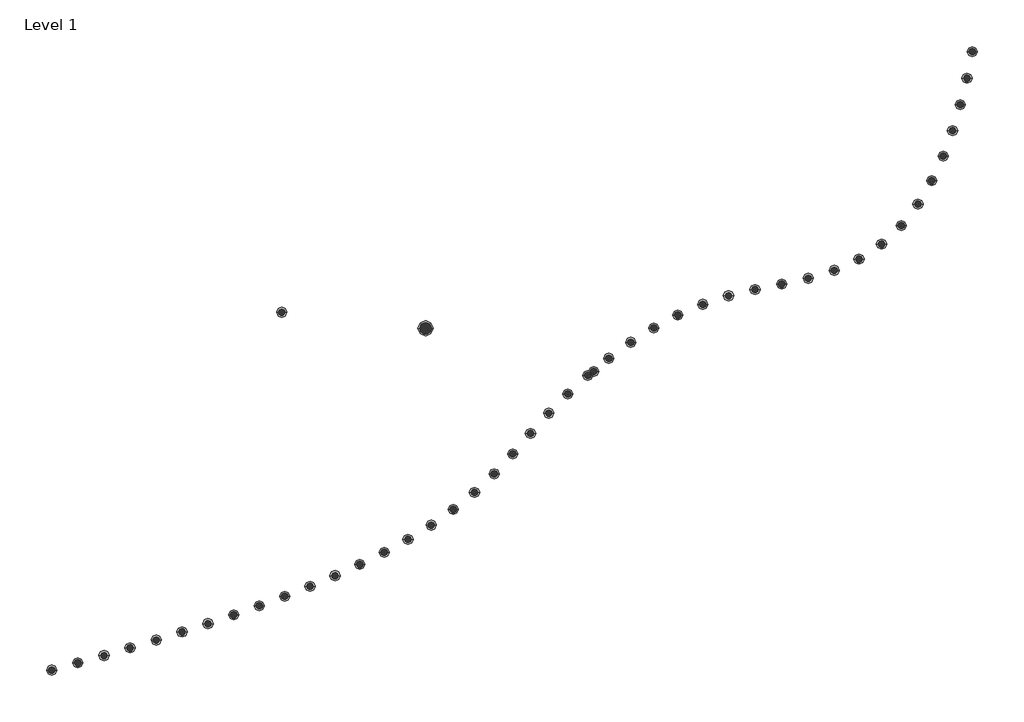
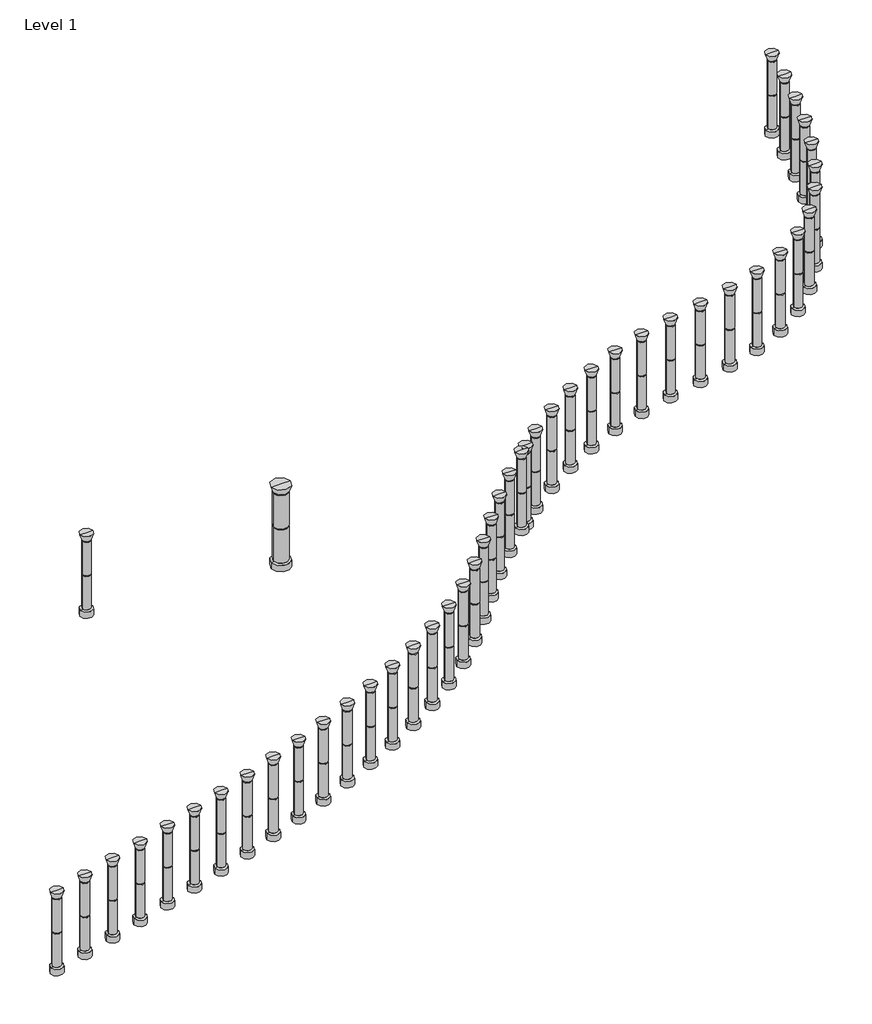
# One storey: 47 columns.
"""IFC4 building model written with IfcOpenShell, lengths in millimetres."""

import ifcopenshell
import ifcopenshell.guid

model = None  # the IFC model being written
_history = None  # IfcOwnerHistory: only IFC2X3 demands one
_inside = {}  # id of a spatial element -> (the spatial element, [elements in it])
_under = {}  # id of a project, library or spatial element -> (it, [spatial elements below it])
_declared = {}  # id of a project -> (the project, [libraries it declares])
_typed = {}  # id of a type object -> (the type object, [elements of that type])
_made_of = {}  # id of a material, layer set ... -> (it, [elements and type objects made of it])


def new_model(schema):
    """Start an empty IFC model of exactly this schema.

    Asked for "IFC4X3", IfcOpenShell would pick the latest addendum, in which some entities
    have other attributes; the version numbers below select the first issue.
    IFC2X3 requires an IfcOwnerHistory on every rooted entity: one is made here for all.
    """
    global model, _history
    if schema == "IFC4X3":
        model = ifcopenshell.file(schema_version=(4, 3, 0, 0))
    else:
        model = ifcopenshell.file(schema=schema)
    _inside.clear()
    _under.clear()
    _declared.clear()
    _typed.clear()
    _made_of.clear()
    _history = None
    if model.schema == "IFC2X3":
        org = make("IfcOrganization", Name="unknown")
        user = make(
            "IfcPersonAndOrganization",
            ThePerson=make("IfcPerson", FamilyName="unknown"),
            TheOrganization=org,
        )
        app = make(
            "IfcApplication",
            ApplicationDeveloper=org,
            Version="unknown",
            ApplicationFullName="unknown",
            ApplicationIdentifier="unknown",
        )
        _history = make(
            "IfcOwnerHistory",
            OwningUser=user,
            OwningApplication=app,
            ChangeAction="ADDED",
            CreationDate=0,
        )
    return model


def make(cls, **values):
    """One entity of the class cls with the attributes given. An attribute that is None is left unset."""
    return model.create_entity(
        cls, **{name: value for name, value in values.items() if value is not None}
    )


def rooted(cls, **values):
    """An entity with a GlobalId (a new one), such as an element, a storey or a relation."""
    return make(cls, GlobalId=ifcopenshell.guid.new(), OwnerHistory=_history, **values)


def si_unit(unit_type, name, prefix=None):
    """IfcSIUnit, for example si_unit("LENGTHUNIT", "METRE", prefix="MILLI")."""
    return make("IfcSIUnit", UnitType=unit_type, Prefix=prefix, Name=name)


def assignment(units):
    """IfcUnitAssignment: the units of a project."""
    return None if units is None else make("IfcUnitAssignment", Units=units)


def point(xyz):
    """IfcCartesianPoint."""
    return None if xyz is None else make("IfcCartesianPoint", Coordinates=xyz)


def direction(xyz):
    """IfcDirection."""
    return None if xyz is None else make("IfcDirection", DirectionRatios=xyz)


def frame(location, z_axis=None, x_axis=None):
    """IfcAxis2Placement3D, a coordinate frame: its origin and axes. An axis left out is left unset."""
    return make(
        "IfcAxis2Placement3D",
        Location=point(location),
        Axis=direction(z_axis),
        RefDirection=direction(x_axis),
    )


def origin():
    """The frame at (0, 0, 0) with its axes left unset."""
    return frame((0.0, 0.0, 0.0))


def origin_with_axes():
    """The frame at (0, 0, 0) with the z axis (0, 0, 1) and the x axis (1, 0, 0) written out."""
    return frame((0.0, 0.0, 0.0), z_axis=(0.0, 0.0, 1.0), x_axis=(1.0, 0.0, 0.0))


def place(relative_to, where):
    """IfcLocalPlacement: puts the frame where relative to a parent placement (None: the world)."""
    return make(
        "IfcLocalPlacement", PlacementRelTo=relative_to, RelativePlacement=where
    )


def context(
    kind, dimensions, precision=None, world=None, true_north=None, identifier=None
):
    """IfcGeometricRepresentationContext, for example the 3D "Model" context."""
    return make(
        "IfcGeometricRepresentationContext",
        ContextIdentifier=identifier,
        ContextType=kind,
        CoordinateSpaceDimension=dimensions,
        Precision=precision,
        WorldCoordinateSystem=world,
        TrueNorth=true_north,
    )


def project(units=None, contexts=None):
    """IfcProject with its units and contexts."""
    return rooted(
        "IfcProject",
        Name="project",
        RepresentationContexts=contexts,
        UnitsInContext=assignment(units),
    )


def spatial(cls, under=None, at=None, **own):
    """A site, building, storey or space (cls), placed at a placement, below another one or the project."""
    s = rooted(cls, ObjectPlacement=at, **own)
    if under is not None:
        _under.setdefault(under.id(), (under, []))[1].append(s)
    return s


def polyline(points):
    """IfcPolyline through the points."""
    return make("IfcPolyline", Points=[point(p) for p in points])


def circle_curve(where, radius):
    """IfcCircle in the frame where."""
    return make("IfcCircle", Position=where, Radius=radius)


def shape(context_of_items, identifier, shape_type, items):
    """IfcShapeRepresentation: the items that make up one representation, for example the "Body"."""
    return make(
        "IfcShapeRepresentation",
        ContextOfItems=context_of_items,
        RepresentationIdentifier=identifier,
        RepresentationType=shape_type,
        Items=items,
    )


def source(mapping_origin, context_of_items, identifier, shape_type, items):
    """IfcRepresentationMap: a shape defined once, which mapped items show again and again."""
    return make(
        "IfcRepresentationMap",
        MappingOrigin=mapping_origin,
        MappedRepresentation=shape(context_of_items, identifier, shape_type, items),
    )


def transform(
    local_origin,
    x_axis=None,
    y_axis=None,
    z_axis=None,
    scale=None,
    scale2=None,
    scale3=None,
    uniform=True,
):
    """IfcCartesianTransformationOperator3D, or its non-uniform kind. x_axis, y_axis, z_axis: its Axis1, 2, 3."""
    if uniform:
        return make(
            "IfcCartesianTransformationOperator3D",
            Axis1=direction(x_axis),
            Axis2=direction(y_axis),
            LocalOrigin=point(local_origin),
            Scale=scale,
            Axis3=direction(z_axis),
        )
    return make(
        "IfcCartesianTransformationOperator3DnonUniform",
        Axis1=direction(x_axis),
        Axis2=direction(y_axis),
        LocalOrigin=point(local_origin),
        Scale=scale,
        Axis3=direction(z_axis),
        Scale2=scale2,
        Scale3=scale3,
    )


def mapped(mapping_source, mapping_target):
    """IfcMappedItem: shows the shape of a source again, moved by a transform."""
    return make(
        "IfcMappedItem", MappingSource=mapping_source, MappingTarget=mapping_target
    )


def made_of(thing, what):
    """Note that an element or type object is made of a material, layer set ...; save() writes the relation."""
    if what is not None:
        _made_of.setdefault(what.id(), (what, []))[1].append(thing)
    return thing


def element(
    cls,
    number,
    at=None,
    inside=None,
    cuts=None,
    type_object=None,
    material=None,
    context=None,
    identifier="Body",
    shape_type=None,
    held_by="IfcProductDefinitionShape",
    body=None,
    shapes=None,
    **own,
):
    """One element of the class cls, such as IfcWall. Its Tag is "e" and its number.

    at: its placement. inside: the storey or other place that contains it. cuts: it is an
    opening in that element (IfcRelVoidsElement). A single representation is given by context,
    identifier, shape_type and body (its items); several are given by shapes. held_by: the class
    of the entity that holds the representations. save() writes the other relations.
    """
    e = rooted(cls, Tag="e%d" % number, ObjectPlacement=at, **own)
    if body is not None:
        shapes = [shape(context, identifier, shape_type, body)]
    if shapes is not None:
        e.Representation = make(held_by, Representations=shapes)
    if inside is not None:
        _inside.setdefault(inside.id(), (inside, []))[1].append(e)
    if cuts is not None:
        rooted(
            "IfcRelVoidsElement", RelatingBuildingElement=cuts, RelatedOpeningElement=e
        )
    if type_object is not None:
        _typed.setdefault(type_object.id(), (type_object, []))[1].append(e)
    return made_of(e, material)


def aggregate(whole, parts):
    """IfcRelAggregates: a whole, such as a stair, and the parts it consists of."""
    return rooted("IfcRelAggregates", RelatingObject=whole, RelatedObjects=parts)


def save(model, path):
    """Write the relations noted so far, then the file.

    IfcRelAggregates (storeys below a building ...), IfcRelContainedInSpatialStructure (elements
    in a storey), IfcRelDefinesByType, IfcRelAssociatesMaterial and IfcRelDeclares: one each for
    every whole, place, type object, material and project.
    """
    for whole, parts in _under.values():
        aggregate(whole, parts)
    for where, things in _inside.values():
        rooted(
            "IfcRelContainedInSpatialStructure",
            RelatedElements=things,
            RelatingStructure=where,
        )
    for kind, things in _typed.values():
        rooted("IfcRelDefinesByType", RelatedObjects=things, RelatingType=kind)
    for what, things in _made_of.values():
        rooted("IfcRelAssociatesMaterial", RelatedObjects=things, RelatingMaterial=what)
    for by, libraries in _declared.values():
        rooted("IfcRelDeclares", RelatingContext=by, RelatedDefinitions=libraries)
    model.write(path)


def plane_surface(at):
    """IfcPlane: the flat surface through the origin of the frame at, square to its z axis."""
    return make("IfcPlane", Position=at)


def cylinder_surface(at, radius):
    """IfcCylindricalSurface: all points at the distance radius from the z axis of the frame at."""
    return make("IfcCylindricalSurface", Position=at, Radius=radius)


def revolved_surface(curve, axis_point, axis_direction):
    """IfcSurfaceOfRevolution: the curve turned about the line through axis_point along axis_direction."""
    return make(
        "IfcSurfaceOfRevolution",
        SweptCurve=make("IfcArbitraryOpenProfileDef", ProfileType="CURVE", Curve=curve),
        AxisPosition=make("IfcAxis1Placement", Location=point(axis_point), Axis=direction(axis_direction)),
    )


def advanced_brep(points, edges, surfaces, faces):
    """IfcAdvancedBrep: a solid bounded by faces that lie on surfaces and meet in shared edges.

    An edge is (start, end): straight between two places in points (the first is 0);
    or (start, end, curve); or (start, end, curve, False) where it runs against its curve.
    A face is (place in surfaces, loops), or (place, loops, False) where it looks against
    its surface's normal. A loop lists edges by number (the first is 1), with a minus sign
    where the edge is run from its end to its start. The first loop is the outer one.
    """
    corners = [point(p) for p in points]
    vertices = [make("IfcVertexPoint", VertexGeometry=c) for c in corners]
    made = []
    for start, end, *more in edges:
        made.append(
            make(
                "IfcEdgeCurve",
                EdgeStart=vertices[start],
                EdgeEnd=vertices[end],
                EdgeGeometry=more[0] if more else make("IfcPolyline", Points=[corners[start], corners[end]]),
                SameSense=more[1] if len(more) > 1 else True,
            )
        )
    hull = []
    for where, loops, *sense in faces:
        bounds = []
        for j, loop in enumerate(loops):
            ring = [make("IfcOrientedEdge", EdgeElement=made[abs(k) - 1], Orientation=k > 0) for k in loop]
            bounds.append(
                make(
                    "IfcFaceOuterBound" if j == 0 else "IfcFaceBound",
                    Bound=make("IfcEdgeLoop", EdgeList=ring),
                    Orientation=True,
                )
            )
        hull.append(make("IfcAdvancedFace", Bounds=bounds, FaceSurface=surfaces[where], SameSense=sense[0] if sense else True))
    return make("IfcAdvancedBrep", Outer=make("IfcClosedShell", CfsFaces=hull))


def column_with_capital_parametric_column_with_capital_56f4d1e8(model_context):
    return source(origin(), model_context, "Body", "AdvancedBrep", [
        advanced_brep(
        [(-300.0, 0.0, 300.0), (300.0, 0.0, 300.0), (300.0, 0.0, 0.0), (-300.0, 0.0, 0.0), (0.0, 0.0, 0.0), (-150.0, 0.0, 300.0), (150.0, 0.0, 300.0), (-150.0, 0.0, 350.0), (150.0, 0.0, 350.0), (-200.0, 0.0, 350.0), (200.0, 0.0, 350.0), (-200.0, 0.0, 1975.0), (200.0, 0.0, 1975.0), (0.0, 0.0, 4000.0), (300.0, 0.0, 4000.0), (-300.0, 0.0, 4000.0), (200.0, 0.0, 3700.0), (-200.0, 0.0, 3700.0), (-150.0, 0.0, 3650.0), (150.0, 0.0, 3650.0), (200.0, 0.0, 3650.0), (-200.0, 0.0, 3650.0), (200.0, 0.0, 2025.0), (-200.0, 0.0, 2025.0), (-150.0, 0.0, 3700.0), (150.0, 0.0, 3700.0), (-150.0, 0.0, 1975.0), (150.0, 0.0, 1975.0), (-150.0, 0.0, 2025.0), (150.0, 0.0, 2025.0)],
        [
            (0, 1, circle_curve(frame((0.0, 0.0, 300.0), z_axis=(0.0, 0.0, -1.0), x_axis=(1.0, 0.0, 0.0)), 300.0)),
            (1, 2),
            (2, 3, circle_curve(origin_with_axes(), 300.0)),
            (3, 0),
            (2, 4),
            (4, 3),
            (2, 3, circle_curve(frame((0.0, 0.0, 0.0), z_axis=(0.0, 0.0, -1.0), x_axis=(1.0, 0.0, 0.0)), 300.0)),
            (1, 0, circle_curve(frame((0.0, 0.0, 300.0), z_axis=(0.0, 0.0, -1.0), x_axis=(1.0, 0.0, 0.0)), 300.0)),
            (5, 6, circle_curve(frame((0.0, 0.0, 300.0), z_axis=(0.0, 0.0, -1.0), x_axis=(1.0, 0.0, 0.0)), 150.0)),
            (6, 1),
            (0, 5),
            (6, 5, circle_curve(frame((0.0, 0.0, 300.0), z_axis=(0.0, 0.0, -1.0), x_axis=(1.0, 0.0, 0.0)), 150.0)),
            (7, 8, circle_curve(frame((0.0, 0.0, 350.0), z_axis=(0.0, 0.0, -1.0), x_axis=(1.0, 0.0, 0.0)), 150.0)),
            (8, 6),
            (5, 7),
            (8, 7, circle_curve(frame((0.0, 0.0, 350.0), z_axis=(0.0, 0.0, -1.0), x_axis=(1.0, 0.0, 0.0)), 150.0)),
            (9, 10, circle_curve(frame((0.0, 0.0, 350.0), z_axis=(0.0, 0.0, -1.0), x_axis=(1.0, 0.0, 0.0)), 200.0)),
            (10, 8),
            (7, 9),
            (10, 9, circle_curve(frame((0.0, 0.0, 350.0), z_axis=(0.0, 0.0, -1.0), x_axis=(1.0, 0.0, 0.0)), 200.0)),
            (11, 12, circle_curve(frame((0.0, 0.0, 1975.0), z_axis=(0.0, 0.0, -1.0), x_axis=(1.0, 0.0, 0.0)), 200.0)),
            (12, 10),
            (9, 11),
            (12, 11, circle_curve(frame((0.0, 0.0, 1975.0), z_axis=(0.0, 0.0, -1.0), x_axis=(1.0, 0.0, 0.0)), 200.0)),
            (13, 14),
            (14, 15, circle_curve(frame((0.0, 0.0, 4000.0), z_axis=(0.0, 0.0, 1.0), x_axis=(1.0, 0.0, 0.0)), 300.0)),
            (15, 13),
            (15, 14, circle_curve(frame((0.0, 0.0, 4000.0), z_axis=(0.0, 0.0, 1.0), x_axis=(1.0, 0.0, 0.0)), 300.0)),
            (14, 16),
            (16, 17, circle_curve(frame((0.0, 0.0, 3700.0), z_axis=(0.0, 0.0, 1.0), x_axis=(1.0, 0.0, 0.0)), 200.0)),
            (17, 15),
            (17, 16, circle_curve(frame((0.0, 0.0, 3700.0), z_axis=(0.0, 0.0, 1.0), x_axis=(1.0, 0.0, 0.0)), 200.0)),
            (18, 19, circle_curve(frame((0.0, 0.0, 3650.0), z_axis=(0.0, 0.0, -1.0), x_axis=(1.0, 0.0, 0.0)), 150.0)),
            (19, 20),
            (20, 21, circle_curve(frame((0.0, 0.0, 3650.0), z_axis=(0.0, 0.0, 1.0), x_axis=(1.0, 0.0, 0.0)), 200.0)),
            (21, 18),
            (20, 22),
            (22, 23, circle_curve(frame((0.0, 0.0, 2025.0), z_axis=(0.0, 0.0, 1.0), x_axis=(1.0, 0.0, 0.0)), 200.0)),
            (23, 21),
            (20, 21, circle_curve(frame((0.0, 0.0, 3650.0), z_axis=(0.0, 0.0, -1.0), x_axis=(1.0, 0.0, 0.0)), 200.0)),
            (23, 22, circle_curve(frame((0.0, 0.0, 2025.0), z_axis=(0.0, 0.0, 1.0), x_axis=(1.0, 0.0, 0.0)), 200.0)),
            (19, 18, circle_curve(frame((0.0, 0.0, 3650.0), z_axis=(0.0, 0.0, -1.0), x_axis=(1.0, 0.0, 0.0)), 150.0)),
            (24, 25, circle_curve(frame((0.0, 0.0, 3700.0), z_axis=(0.0, 0.0, -1.0), x_axis=(1.0, 0.0, 0.0)), 150.0)),
            (25, 19),
            (18, 24),
            (25, 24, circle_curve(frame((0.0, 0.0, 3700.0), z_axis=(0.0, 0.0, -1.0), x_axis=(1.0, 0.0, 0.0)), 150.0)),
            (16, 25),
            (24, 17),
            (26, 27, circle_curve(frame((0.0, 0.0, 1975.0), z_axis=(0.0, 0.0, -1.0), x_axis=(1.0, 0.0, 0.0)), 150.0)),
            (27, 12),
            (11, 26),
            (27, 26, circle_curve(frame((0.0, 0.0, 1975.0), z_axis=(0.0, 0.0, -1.0), x_axis=(1.0, 0.0, 0.0)), 150.0)),
            (28, 29, circle_curve(frame((0.0, 0.0, 2025.0), z_axis=(0.0, 0.0, -1.0), x_axis=(1.0, 0.0, 0.0)), 150.0)),
            (29, 27),
            (26, 28),
            (29, 28, circle_curve(frame((0.0, 0.0, 2025.0), z_axis=(0.0, 0.0, -1.0), x_axis=(1.0, 0.0, 0.0)), 150.0)),
            (22, 29),
            (28, 23),
        ],
        [
            cylinder_surface(frame((0.0, 0.0, 4203.0565088), z_axis=(0.0, 0.0, 1.0), x_axis=(1.0, 0.0, 0.0)), 300.0),
            plane_surface(frame((0.0, 0.0, 0.0), z_axis=(0.0, 0.0, -1.0), x_axis=(1.0, 0.0, 0.0))),
            plane_surface(frame((0.0, 0.0, 300.0), z_axis=(0.0, 0.0, 1.0), x_axis=(1.0, 0.0, 0.0))),
            cylinder_surface(frame((0.0, 0.0, 4203.0565088), z_axis=(0.0, 0.0, 1.0), x_axis=(1.0, 0.0, 0.0)), 150.0),
            plane_surface(frame((0.0, 0.0, 350.0), z_axis=(0.0, 0.0, -1.0), x_axis=(1.0, 0.0, 0.0))),
            cylinder_surface(frame((0.0, 0.0, 4203.0565088), z_axis=(0.0, 0.0, 1.0), x_axis=(1.0, 0.0, 0.0)), 200.0),
            plane_surface(frame((0.0, 0.0, 4000.0), z_axis=(0.0, 0.0, 1.0), x_axis=(1.0, 0.0, 0.0))),
            revolved_surface(polyline([(200.0, 0.0, 3700.0), (300.0, 0.0, 4000.0)]), (0.0, 0.0, 4203.0565088), (0.0, 0.0, 1.0)),
            plane_surface(frame((0.0, 0.0, 3650.0), z_axis=(0.0, 0.0, 1.0), x_axis=(1.0, 0.0, 0.0))),
            plane_surface(frame((0.0, 0.0, 3700.0), z_axis=(0.0, 0.0, -1.0), x_axis=(1.0, 0.0, 0.0))),
            plane_surface(frame((0.0, 0.0, 1975.0), z_axis=(0.0, 0.0, 1.0), x_axis=(1.0, 0.0, 0.0))),
            plane_surface(frame((0.0, 0.0, 2025.0), z_axis=(0.0, 0.0, -1.0), x_axis=(1.0, 0.0, 0.0))),
        ],
        [
            (0, [[1, 2, 3, 4]]),
            (1, [[-3, 5, 6]]),
            (1, [[7, -6, -5]]),
            (0, [[8, -4, -7, -2]]),
            (2, [[9, 10, -1, 11]]),
            (2, [[12, -11, -8, -10]]),
            (3, [[13, 14, -9, 15]]),
            (3, [[16, -15, -12, -14]]),
            (4, [[17, 18, -13, 19]]),
            (4, [[20, -19, -16, -18]]),
            (5, [[21, 22, -17, 23]]),
            (5, [[24, -23, -20, -22]]),
            (6, [[25, 26, 27]]),
            (6, [[-27, 28, -25]]),
            (7, [[-26, 29, 30, 31]]),
            (7, [[-28, -31, 32, -29]]),
            (8, [[33, 34, 35, 36]]),
            (5, [[-35, 37, 38, 39]]),
            (5, [[40, -39, 41, -37]]),
            (8, [[42, -36, -40, -34]]),
            (3, [[43, 44, -33, 45]]),
            (3, [[46, -45, -42, -44]]),
            (9, [[-30, 47, -43, 48]]),
            (9, [[-32, -48, -46, -47]]),
            (10, [[49, 50, -21, 51]]),
            (10, [[52, -51, -24, -50]]),
            (3, [[53, 54, -49, 55]]),
            (3, [[56, -55, -52, -54]]),
            (11, [[-38, 57, -53, 58]]),
            (11, [[-41, -58, -56, -57]]),
        ],
    ),
    ])


def column_with_capital_parametric_column_with_capital_d26f2c8e(model_context):
    return source(origin(), model_context, "Body", "AdvancedBrep", [
        advanced_brep(
        [(-450.0, 0.0, 300.0), (450.0, 0.0, 300.0), (450.0, 0.0, 0.0), (-450.0, 0.0, 0.0), (0.0, 0.0, 0.0), (-300.0, 0.0, 300.0), (300.0, 0.0, 300.0), (-300.0, 0.0, 350.0), (300.0, 0.0, 350.0), (-350.0, 0.0, 350.0), (350.0, 0.0, 350.0), (-350.0, 0.0, 1975.0), (350.0, 0.0, 1975.0), (0.0, 0.0, 4000.0), (450.0, 0.0, 4000.0), (-450.0, 0.0, 4000.0), (350.0, 0.0, 3700.0), (-350.0, 0.0, 3700.0), (-300.0, 0.0, 3650.0), (300.0, 0.0, 3650.0), (350.0, 0.0, 3650.0), (-350.0, 0.0, 3650.0), (350.0, 0.0, 2025.0), (-350.0, 0.0, 2025.0), (-300.0, 0.0, 3700.0), (300.0, 0.0, 3700.0), (-300.0, 0.0, 1975.0), (300.0, 0.0, 1975.0), (-300.0, 0.0, 2025.0), (300.0, 0.0, 2025.0)],
        [
            (0, 1, circle_curve(frame((0.0, 0.0, 300.0), z_axis=(0.0, 0.0, -1.0), x_axis=(1.0, 0.0, 0.0)), 450.0)),
            (1, 2),
            (2, 3, circle_curve(origin_with_axes(), 450.0)),
            (3, 0),
            (2, 4),
            (4, 3),
            (2, 3, circle_curve(frame((0.0, 0.0, 0.0), z_axis=(0.0, 0.0, -1.0), x_axis=(1.0, 0.0, 0.0)), 450.0)),
            (1, 0, circle_curve(frame((0.0, 0.0, 300.0), z_axis=(0.0, 0.0, -1.0), x_axis=(1.0, 0.0, 0.0)), 450.0)),
            (5, 6, circle_curve(frame((0.0, 0.0, 300.0), z_axis=(0.0, 0.0, -1.0), x_axis=(1.0, 0.0, 0.0)), 300.0)),
            (6, 1),
            (0, 5),
            (6, 5, circle_curve(frame((0.0, 0.0, 300.0), z_axis=(0.0, 0.0, -1.0), x_axis=(1.0, 0.0, 0.0)), 300.0)),
            (7, 8, circle_curve(frame((0.0, 0.0, 350.0), z_axis=(0.0, 0.0, -1.0), x_axis=(1.0, 0.0, 0.0)), 300.0)),
            (8, 6),
            (5, 7),
            (8, 7, circle_curve(frame((0.0, 0.0, 350.0), z_axis=(0.0, 0.0, -1.0), x_axis=(1.0, 0.0, 0.0)), 300.0)),
            (9, 10, circle_curve(frame((0.0, 0.0, 350.0), z_axis=(0.0, 0.0, -1.0), x_axis=(1.0, 0.0, 0.0)), 350.0)),
            (10, 8),
            (7, 9),
            (10, 9, circle_curve(frame((0.0, 0.0, 350.0), z_axis=(0.0, 0.0, -1.0), x_axis=(1.0, 0.0, 0.0)), 350.0)),
            (11, 12, circle_curve(frame((0.0, 0.0, 1975.0), z_axis=(0.0, 0.0, -1.0), x_axis=(1.0, 0.0, 0.0)), 350.0)),
            (12, 10),
            (9, 11),
            (12, 11, circle_curve(frame((0.0, 0.0, 1975.0), z_axis=(0.0, 0.0, -1.0), x_axis=(1.0, 0.0, 0.0)), 350.0)),
            (13, 14),
            (14, 15, circle_curve(frame((0.0, 0.0, 4000.0), z_axis=(0.0, 0.0, 1.0), x_axis=(1.0, 0.0, 0.0)), 450.0)),
            (15, 13),
            (15, 14, circle_curve(frame((0.0, 0.0, 4000.0), z_axis=(0.0, 0.0, 1.0), x_axis=(1.0, 0.0, 0.0)), 450.0)),
            (14, 16),
            (16, 17, circle_curve(frame((0.0, 0.0, 3700.0), z_axis=(0.0, 0.0, 1.0), x_axis=(1.0, 0.0, 0.0)), 350.0)),
            (17, 15),
            (17, 16, circle_curve(frame((0.0, 0.0, 3700.0), z_axis=(0.0, 0.0, 1.0), x_axis=(1.0, 0.0, 0.0)), 350.0)),
            (18, 19, circle_curve(frame((0.0, 0.0, 3650.0), z_axis=(0.0, 0.0, -1.0), x_axis=(1.0, 0.0, 0.0)), 300.0)),
            (19, 20),
            (20, 21, circle_curve(frame((0.0, 0.0, 3650.0), z_axis=(0.0, 0.0, 1.0), x_axis=(1.0, 0.0, 0.0)), 350.0)),
            (21, 18),
            (20, 22),
            (22, 23, circle_curve(frame((0.0, 0.0, 2025.0), z_axis=(0.0, 0.0, 1.0), x_axis=(1.0, 0.0, 0.0)), 350.0)),
            (23, 21),
            (20, 21, circle_curve(frame((0.0, 0.0, 3650.0), z_axis=(0.0, 0.0, -1.0), x_axis=(1.0, 0.0, 0.0)), 350.0)),
            (23, 22, circle_curve(frame((0.0, 0.0, 2025.0), z_axis=(0.0, 0.0, 1.0), x_axis=(1.0, 0.0, 0.0)), 350.0)),
            (19, 18, circle_curve(frame((0.0, 0.0, 3650.0), z_axis=(0.0, 0.0, -1.0), x_axis=(1.0, 0.0, 0.0)), 300.0)),
            (24, 25, circle_curve(frame((0.0, 0.0, 3700.0), z_axis=(0.0, 0.0, -1.0), x_axis=(1.0, 0.0, 0.0)), 300.0)),
            (25, 19),
            (18, 24),
            (25, 24, circle_curve(frame((0.0, 0.0, 3700.0), z_axis=(0.0, 0.0, -1.0), x_axis=(1.0, 0.0, 0.0)), 300.0)),
            (16, 25),
            (24, 17),
            (26, 27, circle_curve(frame((0.0, 0.0, 1975.0), z_axis=(0.0, 0.0, -1.0), x_axis=(1.0, 0.0, 0.0)), 300.0)),
            (27, 12),
            (11, 26),
            (27, 26, circle_curve(frame((0.0, 0.0, 1975.0), z_axis=(0.0, 0.0, -1.0), x_axis=(1.0, 0.0, 0.0)), 300.0)),
            (28, 29, circle_curve(frame((0.0, 0.0, 2025.0), z_axis=(0.0, 0.0, -1.0), x_axis=(1.0, 0.0, 0.0)), 300.0)),
            (29, 27),
            (26, 28),
            (29, 28, circle_curve(frame((0.0, 0.0, 2025.0), z_axis=(0.0, 0.0, -1.0), x_axis=(1.0, 0.0, 0.0)), 300.0)),
            (22, 29),
            (28, 23),
        ],
        [
            cylinder_surface(frame((0.0, 0.0, 4203.0565088), z_axis=(0.0, 0.0, 1.0), x_axis=(1.0, 0.0, 0.0)), 450.0),
            plane_surface(frame((0.0, 0.0, 0.0), z_axis=(0.0, 0.0, -1.0), x_axis=(1.0, 0.0, 0.0))),
            plane_surface(frame((0.0, 0.0, 300.0), z_axis=(0.0, 0.0, 1.0), x_axis=(1.0, 0.0, 0.0))),
            cylinder_surface(frame((0.0, 0.0, 4203.0565088), z_axis=(0.0, 0.0, 1.0), x_axis=(1.0, 0.0, 0.0)), 300.0),
            plane_surface(frame((0.0, 0.0, 350.0), z_axis=(0.0, 0.0, -1.0), x_axis=(1.0, 0.0, 0.0))),
            cylinder_surface(frame((0.0, 0.0, 4203.0565088), z_axis=(0.0, 0.0, 1.0), x_axis=(1.0, 0.0, 0.0)), 350.0),
            plane_surface(frame((0.0, 0.0, 4000.0), z_axis=(0.0, 0.0, 1.0), x_axis=(1.0, 0.0, 0.0))),
            revolved_surface(polyline([(350.0, 0.0, 3700.0), (450.0, 0.0, 4000.0)]), (0.0, 0.0, 4203.0565088), (0.0, 0.0, 1.0)),
            plane_surface(frame((0.0, 0.0, 3650.0), z_axis=(0.0, 0.0, 1.0), x_axis=(1.0, 0.0, 0.0))),
            plane_surface(frame((0.0, 0.0, 3700.0), z_axis=(0.0, 0.0, -1.0), x_axis=(1.0, 0.0, 0.0))),
            plane_surface(frame((0.0, 0.0, 1975.0), z_axis=(0.0, 0.0, 1.0), x_axis=(1.0, 0.0, 0.0))),
            plane_surface(frame((0.0, 0.0, 2025.0), z_axis=(0.0, 0.0, -1.0), x_axis=(1.0, 0.0, 0.0))),
        ],
        [
            (0, [[1, 2, 3, 4]]),
            (1, [[-3, 5, 6]]),
            (1, [[7, -6, -5]]),
            (0, [[8, -4, -7, -2]]),
            (2, [[9, 10, -1, 11]]),
            (2, [[12, -11, -8, -10]]),
            (3, [[13, 14, -9, 15]]),
            (3, [[16, -15, -12, -14]]),
            (4, [[17, 18, -13, 19]]),
            (4, [[20, -19, -16, -18]]),
            (5, [[21, 22, -17, 23]]),
            (5, [[24, -23, -20, -22]]),
            (6, [[25, 26, 27]]),
            (6, [[-27, 28, -25]]),
            (7, [[-26, 29, 30, 31]]),
            (7, [[-28, -31, 32, -29]]),
            (8, [[33, 34, 35, 36]]),
            (5, [[-35, 37, 38, 39]]),
            (5, [[40, -39, 41, -37]]),
            (8, [[42, -36, -40, -34]]),
            (3, [[43, 44, -33, 45]]),
            (3, [[46, -45, -42, -44]]),
            (9, [[-30, 47, -43, 48]]),
            (9, [[-32, -48, -46, -47]]),
            (10, [[49, 50, -21, 51]]),
            (10, [[52, -51, -24, -50]]),
            (3, [[53, 54, -49, 55]]),
            (3, [[56, -55, -52, -54]]),
            (11, [[-38, 57, -53, 58]]),
            (11, [[-41, -58, -56, -57]]),
        ],
    ),
    ])


model = new_model("IFC4")

# Units and contexts
model_context = context("Model", 3, world=origin())
ifc_project = project(units=[si_unit("LENGTHUNIT", "METRE", prefix="MILLI")], contexts=[model_context])

# Site, building, storey
site = spatial("IfcSite", under=ifc_project)
building = spatial("IfcBuilding", under=site)
storey = spatial("IfcBuildingStorey", under=building, Name="Level 1", Elevation=0.0)

# Columns
placement = place(None, origin())
column_with_capital_parametric_column_with_capital_shape = column_with_capital_parametric_column_with_capital_56f4d1e8(model_context)
element("IfcColumn", 1, ObjectType="Column-with-capital-parametric : Column-with-capital-parametric", at=placement, inside=storey, context=model_context, shape_type="MappedRepresentation", body=[
    mapped(column_with_capital_parametric_column_with_capital_shape, transform((-8152.9672643, 3520.2375334, 0.0), x_axis=(1.0, 0.0, 0.0), y_axis=(0.0, 1.0, 0.0), z_axis=(0.0, 0.0, 1.0))),
])
element("IfcColumn", 2, ObjectType="Column-with-capital-parametric : Column-with-capital-parametric", at=placement, inside=storey, context=model_context, shape_type="MappedRepresentation", body=[
    mapped(column_with_capital_parametric_column_with_capital_shape, transform((10210.6062863, 37.4908255, 0.0), x_axis=(1.0, 0.0, 0.0), y_axis=(0.0, 1.0, 0.0), z_axis=(0.0, 0.0, 1.0))),
])
element("IfcColumn", 3, ObjectType="Column-with-capital-parametric : Column-with-capital-parametric", at=placement, inside=storey, context=model_context, shape_type="MappedRepresentation", body=[
    mapped(column_with_capital_parametric_column_with_capital_shape, transform((-21695.5106489, -17560.5132214, 0.0), x_axis=(1.0, 0.0, 0.0), y_axis=(0.0, 1.0, 0.0), z_axis=(0.0, 0.0, 1.0))),
])
element("IfcColumn", 4, ObjectType="Column-with-capital-parametric : Column-with-capital-parametric", at=placement, inside=storey, context=model_context, shape_type="MappedRepresentation", body=[
    mapped(column_with_capital_parametric_column_with_capital_shape, transform((-20152.8357635, -17136.0795147, 0.0), x_axis=(1.0, 0.0, 0.0), y_axis=(0.0, 1.0, 0.0), z_axis=(0.0, 0.0, 1.0))),
])
element("IfcColumn", 5, ObjectType="Column-with-capital-parametric : Column-with-capital-parametric", at=placement, inside=storey, context=model_context, shape_type="MappedRepresentation", body=[
    mapped(column_with_capital_parametric_column_with_capital_shape, transform((-18613.2863052, -16700.4477151, 0.0), x_axis=(1.0, 0.0, 0.0), y_axis=(0.0, 1.0, 0.0), z_axis=(0.0, 0.0, 1.0))),
])
element("IfcColumn", 6, ObjectType="Column-with-capital-parametric : Column-with-capital-parametric", at=placement, inside=storey, context=model_context, shape_type="MappedRepresentation", body=[
    mapped(column_with_capital_parametric_column_with_capital_shape, transform((-17077.2822328, -16252.47864, 0.0), x_axis=(1.0, 0.0, 0.0), y_axis=(0.0, 1.0, 0.0), z_axis=(0.0, 0.0, 1.0))),
])
element("IfcColumn", 7, ObjectType="Column-with-capital-parametric : Column-with-capital-parametric", at=placement, inside=storey, context=model_context, shape_type="MappedRepresentation", body=[
    mapped(column_with_capital_parametric_column_with_capital_shape, transform((-15545.3305484, -15790.8454601, 0.0), x_axis=(1.0, 0.0, 0.0), y_axis=(0.0, 1.0, 0.0), z_axis=(0.0, 0.0, 1.0))),
])
element("IfcColumn", 8, ObjectType="Column-with-capital-parametric : Column-with-capital-parametric", at=placement, inside=storey, context=model_context, shape_type="MappedRepresentation", body=[
    mapped(column_with_capital_parametric_column_with_capital_shape, transform((-14018.0499467, -15313.9908757, 0.0), x_axis=(1.0, 0.0, 0.0), y_axis=(0.0, 1.0, 0.0), z_axis=(0.0, 0.0, 1.0))),
])
element("IfcColumn", 9, ObjectType="Column-with-capital-parametric : Column-with-capital-parametric", at=placement, inside=storey, context=model_context, shape_type="MappedRepresentation", body=[
    mapped(column_with_capital_parametric_column_with_capital_shape, transform((-12496.2043862, -14820.071923, 0.0), x_axis=(1.0, 0.0, 0.0), y_axis=(0.0, 1.0, 0.0), z_axis=(0.0, 0.0, 1.0))),
])
element("IfcColumn", 10, ObjectType="Column-with-capital-parametric : Column-with-capital-parametric", at=placement, inside=storey, context=model_context, shape_type="MappedRepresentation", body=[
    mapped(column_with_capital_parametric_column_with_capital_shape, transform((-10980.7495159, -14306.8882406, 0.0), x_axis=(1.0, 0.0, 0.0), y_axis=(0.0, 1.0, 0.0), z_axis=(0.0, 0.0, 1.0))),
])
element("IfcColumn", 11, ObjectType="Column-with-capital-parametric : Column-with-capital-parametric", at=placement, inside=storey, context=model_context, shape_type="MappedRepresentation", body=[
    mapped(column_with_capital_parametric_column_with_capital_shape, transform((-9472.8979095, -13771.7881682, 0.0), x_axis=(1.0, 0.0, 0.0), y_axis=(0.0, 1.0, 0.0), z_axis=(0.0, 0.0, 1.0))),
])
element("IfcColumn", 12, ObjectType="Column-with-capital-parametric : Column-with-capital-parametric", at=placement, inside=storey, context=model_context, shape_type="MappedRepresentation", body=[
    mapped(column_with_capital_parametric_column_with_capital_shape, transform((-7974.2122248, -13211.5452838, 0.0), x_axis=(1.0, 0.0, 0.0), y_axis=(0.0, 1.0, 0.0), z_axis=(0.0, 0.0, 1.0))),
])
element("IfcColumn", 13, ObjectType="Column-with-capital-parametric : Column-with-capital-parametric", at=placement, inside=storey, context=model_context, shape_type="MappedRepresentation", body=[
    mapped(column_with_capital_parametric_column_with_capital_shape, transform((-6486.7402876, -12622.1962117, 0.0), x_axis=(1.0, 0.0, 0.0), y_axis=(0.0, 1.0, 0.0), z_axis=(0.0, 0.0, 1.0))),
])
element("IfcColumn", 14, ObjectType="Column-with-capital-parametric : Column-with-capital-parametric", at=placement, inside=storey, context=model_context, shape_type="MappedRepresentation", body=[
    mapped(column_with_capital_parametric_column_with_capital_shape, transform((-5013.2134877, -11998.8300086, 0.0), x_axis=(1.0, 0.0, 0.0), y_axis=(0.0, 1.0, 0.0), z_axis=(0.0, 0.0, 1.0))),
])
element("IfcColumn", 15, ObjectType="Column-with-capital-parametric : Column-with-capital-parametric", at=placement, inside=storey, context=model_context, shape_type="MappedRepresentation", body=[
    mapped(column_with_capital_parametric_column_with_capital_shape, transform((-3557.3399805, -11335.3238671, 0.0), x_axis=(1.0, 0.0, 0.0), y_axis=(0.0, 1.0, 0.0), z_axis=(0.0, 0.0, 1.0))),
])
element("IfcColumn", 16, ObjectType="Column-with-capital-parametric : Column-with-capital-parametric", at=placement, inside=storey, context=model_context, shape_type="MappedRepresentation", body=[
    mapped(column_with_capital_parametric_column_with_capital_shape, transform((-2124.2342269, -10624.0396541, 0.0), x_axis=(1.0, 0.0, 0.0), y_axis=(0.0, 1.0, 0.0), z_axis=(0.0, 0.0, 1.0))),
])
element("IfcColumn", 17, ObjectType="Column-with-capital-parametric : Column-with-capital-parametric", at=placement, inside=storey, context=model_context, shape_type="MappedRepresentation", body=[
    mapped(column_with_capital_parametric_column_with_capital_shape, transform((-721.0192677, -9855.5579132, 0.0), x_axis=(1.0, 0.0, 0.0), y_axis=(0.0, 1.0, 0.0), z_axis=(0.0, 0.0, 1.0))),
])
element("IfcColumn", 18, ObjectType="Column-with-capital-parametric : Column-with-capital-parametric", at=placement, inside=storey, context=model_context, shape_type="MappedRepresentation", body=[
    mapped(column_with_capital_parametric_column_with_capital_shape, transform((642.440057, -9018.6931372, 0.0), x_axis=(1.0, 0.0, 0.0), y_axis=(0.0, 1.0, 0.0), z_axis=(0.0, 0.0, 1.0))),
])
element("IfcColumn", 19, ObjectType="Column-with-capital-parametric : Column-with-capital-parametric", at=placement, inside=storey, context=model_context, shape_type="MappedRepresentation", body=[
    mapped(column_with_capital_parametric_column_with_capital_shape, transform((1953.0441744, -8101.4178308, 0.0), x_axis=(1.0, 0.0, 0.0), y_axis=(0.0, 1.0, 0.0), z_axis=(0.0, 0.0, 1.0))),
])
element("IfcColumn", 20, ObjectType="Column-with-capital-parametric : Column-with-capital-parametric", at=placement, inside=storey, context=model_context, shape_type="MappedRepresentation", body=[
    mapped(column_with_capital_parametric_column_with_capital_shape, transform((3195.5523811, -7093.9574146, 0.0), x_axis=(1.0, 0.0, 0.0), y_axis=(0.0, 1.0, 0.0), z_axis=(0.0, 0.0, 1.0))),
])
element("IfcColumn", 21, ObjectType="Column-with-capital-parametric : Column-with-capital-parametric", at=placement, inside=storey, context=model_context, shape_type="MappedRepresentation", body=[
    mapped(column_with_capital_parametric_column_with_capital_shape, transform((4358.3832858, -5995.4835983, 0.0), x_axis=(1.0, 0.0, 0.0), y_axis=(0.0, 1.0, 0.0), z_axis=(0.0, 0.0, 1.0))),
])
element("IfcColumn", 22, ObjectType="Column-with-capital-parametric : Column-with-capital-parametric", at=placement, inside=storey, context=model_context, shape_type="MappedRepresentation", body=[
    mapped(column_with_capital_parametric_column_with_capital_shape, transform((5446.9482545, -4823.1286411, 0.0), x_axis=(1.0, 0.0, 0.0), y_axis=(0.0, 1.0, 0.0), z_axis=(0.0, 0.0, 1.0))),
])
element("IfcColumn", 23, ObjectType="Column-with-capital-parametric : Column-with-capital-parametric", at=placement, inside=storey, context=model_context, shape_type="MappedRepresentation", body=[
    mapped(column_with_capital_parametric_column_with_capital_shape, transform((6497.1953955, -3616.0848621, 0.0), x_axis=(1.0, 0.0, 0.0), y_axis=(0.0, 1.0, 0.0), z_axis=(0.0, 0.0, 1.0))),
])
element("IfcColumn", 24, ObjectType="Column-with-capital-parametric : Column-with-capital-parametric", at=placement, inside=storey, context=model_context, shape_type="MappedRepresentation", body=[
    mapped(column_with_capital_parametric_column_with_capital_shape, transform((7567.513641, -2426.9364406, 0.0), x_axis=(1.0, 0.0, 0.0), y_axis=(0.0, 1.0, 0.0), z_axis=(0.0, 0.0, 1.0))),
])
element("IfcColumn", 25, ObjectType="Column-with-capital-parametric : Column-with-capital-parametric", at=placement, inside=storey, context=model_context, shape_type="MappedRepresentation", body=[
    mapped(column_with_capital_parametric_column_with_capital_shape, transform((8691.0741079, -1288.0295243, 0.0), x_axis=(1.0, 0.0, 0.0), y_axis=(0.0, 1.0, 0.0), z_axis=(0.0, 0.0, 1.0))),
])
element("IfcColumn", 26, ObjectType="Column-with-capital-parametric : Column-with-capital-parametric", at=placement, inside=storey, context=model_context, shape_type="MappedRepresentation", body=[
    mapped(column_with_capital_parametric_column_with_capital_shape, transform((9870.5455614, -207.1674867, 0.0), x_axis=(1.0, 0.0, 0.0), y_axis=(0.0, 1.0, 0.0), z_axis=(0.0, 0.0, 1.0))),
])
element("IfcColumn", 27, ObjectType="Column-with-capital-parametric : Column-with-capital-parametric", at=placement, inside=storey, context=model_context, shape_type="MappedRepresentation", body=[
    mapped(column_with_capital_parametric_column_with_capital_shape, transform((11107.2505627, 807.6558535, 0.0), x_axis=(1.0, 0.0, 0.0), y_axis=(0.0, 1.0, 0.0), z_axis=(0.0, 0.0, 1.0))),
])
element("IfcColumn", 28, ObjectType="Column-with-capital-parametric : Column-with-capital-parametric", at=placement, inside=storey, context=model_context, shape_type="MappedRepresentation", body=[
    mapped(column_with_capital_parametric_column_with_capital_shape, transform((12402.3540552, 1746.7348667, 0.0), x_axis=(1.0, 0.0, 0.0), y_axis=(0.0, 1.0, 0.0), z_axis=(0.0, 0.0, 1.0))),
])
element("IfcColumn", 29, ObjectType="Column-with-capital-parametric : Column-with-capital-parametric", at=placement, inside=storey, context=model_context, shape_type="MappedRepresentation", body=[
    mapped(column_with_capital_parametric_column_with_capital_shape, transform((13756.3748078, 2598.5619095, 0.0), x_axis=(1.0, 0.0, 0.0), y_axis=(0.0, 1.0, 0.0), z_axis=(0.0, 0.0, 1.0))),
])
element("IfcColumn", 30, ObjectType="Column-with-capital-parametric : Column-with-capital-parametric", at=placement, inside=storey, context=model_context, shape_type="MappedRepresentation", body=[
    mapped(column_with_capital_parametric_column_with_capital_shape, transform((15168.5666566, 3349.8776443, 0.0), x_axis=(1.0, 0.0, 0.0), y_axis=(0.0, 1.0, 0.0), z_axis=(0.0, 0.0, 1.0))),
])
element("IfcColumn", 31, ObjectType="Column-with-capital-parametric : Column-with-capital-parametric", at=placement, inside=storey, context=model_context, shape_type="MappedRepresentation", body=[
    mapped(column_with_capital_parametric_column_with_capital_shape, transform((16636.1662169, 3986.0050122, 0.0), x_axis=(1.0, 0.0, 0.0), y_axis=(0.0, 1.0, 0.0), z_axis=(0.0, 0.0, 1.0))),
])
element("IfcColumn", 32, ObjectType="Column-with-capital-parametric : Column-with-capital-parametric", at=placement, inside=storey, context=model_context, shape_type="MappedRepresentation", body=[
    mapped(column_with_capital_parametric_column_with_capital_shape, transform((18153.5894562, 4491.6346687, 0.0), x_axis=(1.0, 0.0, 0.0), y_axis=(0.0, 1.0, 0.0), z_axis=(0.0, 0.0, 1.0))),
])
element("IfcColumn", 33, ObjectType="Column-with-capital-parametric : Column-with-capital-parametric", at=placement, inside=storey, context=model_context, shape_type="MappedRepresentation", body=[
    mapped(column_with_capital_parametric_column_with_capital_shape, transform((19709.056907, 4865.0829155, 0.0), x_axis=(1.0, 0.0, 0.0), y_axis=(0.0, 1.0, 0.0), z_axis=(0.0, 0.0, 1.0))),
])
element("IfcColumn", 34, ObjectType="Column-with-capital-parametric : Column-with-capital-parametric", at=placement, inside=storey, context=model_context, shape_type="MappedRepresentation", body=[
    mapped(column_with_capital_parametric_column_with_capital_shape, transform((21278.1464693, 5178.022368, 0.0), x_axis=(1.0, 0.0, 0.0), y_axis=(0.0, 1.0, 0.0), z_axis=(0.0, 0.0, 1.0))),
])
element("IfcColumn", 35, ObjectType="Column-with-capital-parametric : Column-with-capital-parametric", at=placement, inside=storey, context=model_context, shape_type="MappedRepresentation", body=[
    mapped(column_with_capital_parametric_column_with_capital_shape, transform((22840.1478184, 5523.8698583, 0.0), x_axis=(1.0, 0.0, 0.0), y_axis=(0.0, 1.0, 0.0), z_axis=(0.0, 0.0, 1.0))),
])
element("IfcColumn", 36, ObjectType="Column-with-capital-parametric : Column-with-capital-parametric", at=placement, inside=storey, context=model_context, shape_type="MappedRepresentation", body=[
    mapped(column_with_capital_parametric_column_with_capital_shape, transform((24370.1647548, 5989.393128, 0.0), x_axis=(1.0, 0.0, 0.0), y_axis=(0.0, 1.0, 0.0), z_axis=(0.0, 0.0, 1.0))),
])
element("IfcColumn", 37, ObjectType="Column-with-capital-parametric : Column-with-capital-parametric", at=placement, inside=storey, context=model_context, shape_type="MappedRepresentation", body=[
    mapped(column_with_capital_parametric_column_with_capital_shape, transform((25827.5337162, 6646.1318062, 0.0), x_axis=(1.0, 0.0, 0.0), y_axis=(0.0, 1.0, 0.0), z_axis=(0.0, 0.0, 1.0))),
])
element("IfcColumn", 38, ObjectType="Column-with-capital-parametric : Column-with-capital-parametric", at=placement, inside=storey, context=model_context, shape_type="MappedRepresentation", body=[
    mapped(column_with_capital_parametric_column_with_capital_shape, transform((27158.882467, 7529.9877286, 0.0), x_axis=(1.0, 0.0, 0.0), y_axis=(0.0, 1.0, 0.0), z_axis=(0.0, 0.0, 1.0))),
])
element("IfcColumn", 39, ObjectType="Column-with-capital-parametric : Column-with-capital-parametric", at=placement, inside=storey, context=model_context, shape_type="MappedRepresentation", body=[
    mapped(column_with_capital_parametric_column_with_capital_shape, transform((28320.8114697, 8627.281215, 0.0), x_axis=(1.0, 0.0, 0.0), y_axis=(0.0, 1.0, 0.0), z_axis=(0.0, 0.0, 1.0))),
])
element("IfcColumn", 40, ObjectType="Column-with-capital-parametric : Column-with-capital-parametric", at=placement, inside=storey, context=model_context, shape_type="MappedRepresentation", body=[
    mapped(column_with_capital_parametric_column_with_capital_shape, transform((29300.6314706, 9890.4896657, 0.0), x_axis=(1.0, 0.0, 0.0), y_axis=(0.0, 1.0, 0.0), z_axis=(0.0, 0.0, 1.0))),
])
element("IfcColumn", 41, ObjectType="Column-with-capital-parametric : Column-with-capital-parametric", at=placement, inside=storey, context=model_context, shape_type="MappedRepresentation", body=[
    mapped(column_with_capital_parametric_column_with_capital_shape, transform((30112.9201467, 11267.9771671, 0.0), x_axis=(1.0, 0.0, 0.0), y_axis=(0.0, 1.0, 0.0), z_axis=(0.0, 0.0, 1.0))),
])
element("IfcColumn", 42, ObjectType="Column-with-capital-parametric : Column-with-capital-parametric", at=placement, inside=storey, context=model_context, shape_type="MappedRepresentation", body=[
    mapped(column_with_capital_parametric_column_with_capital_shape, transform((30783.5379399, 12720.0819922, 0.0), x_axis=(1.0, 0.0, 0.0), y_axis=(0.0, 1.0, 0.0), z_axis=(0.0, 0.0, 1.0))),
])
element("IfcColumn", 43, ObjectType="Column-with-capital-parametric : Column-with-capital-parametric", at=placement, inside=storey, context=model_context, shape_type="MappedRepresentation", body=[
    mapped(column_with_capital_parametric_column_with_capital_shape, transform((31338.3722481, 14220.4594346, 0.0), x_axis=(1.0, 0.0, 0.0), y_axis=(0.0, 1.0, 0.0), z_axis=(0.0, 0.0, 1.0))),
])
element("IfcColumn", 44, ObjectType="Column-with-capital-parametric : Column-with-capital-parametric", at=placement, inside=storey, context=model_context, shape_type="MappedRepresentation", body=[
    mapped(column_with_capital_parametric_column_with_capital_shape, transform((31799.2094569, 15752.4444139, 0.0), x_axis=(1.0, 0.0, 0.0), y_axis=(0.0, 1.0, 0.0), z_axis=(0.0, 0.0, 1.0))),
])
element("IfcColumn", 45, ObjectType="Column-with-capital-parametric : Column-with-capital-parametric", at=placement, inside=storey, context=model_context, shape_type="MappedRepresentation", body=[
    mapped(column_with_capital_parametric_column_with_capital_shape, transform((32183.2675895, 17305.5291336, 0.0), x_axis=(1.0, 0.0, 0.0), y_axis=(0.0, 1.0, 0.0), z_axis=(0.0, 0.0, 1.0))),
])
element("IfcColumn", 46, ObjectType="Column-with-capital-parametric : Column-with-capital-parametric", at=placement, inside=storey, context=model_context, shape_type="MappedRepresentation", body=[
    mapped(column_with_capital_parametric_column_with_capital_shape, transform((32503.9019528, 18872.9804629, 0.0), x_axis=(1.0, 0.0, 0.0), y_axis=(0.0, 1.0, 0.0), z_axis=(0.0, 0.0, 1.0))),
])
column_with_capital_parametric_column_with_capital_2_shape = column_with_capital_parametric_column_with_capital_d26f2c8e(model_context)
element("IfcColumn", 47, ObjectType="Column-with-capital-parametric : Column-with-capital-parametric", at=placement, inside=storey, context=model_context, shape_type="MappedRepresentation", body=[
    mapped(column_with_capital_parametric_column_with_capital_2_shape, transform((316.4395026, 2570.3975222, 0.0), x_axis=(1.0, 0.0, 0.0), y_axis=(0.0, 1.0, 0.0), z_axis=(0.0, 0.0, 1.0))),
])

save(model, "model.ifc")

# Revit data of these elements
# Project information
#   Project Issue Date = "Issue Date"
#   Project Status = "Project Status"
#   Client Name = "Owner"
#   Project Address = "Enter address here"
#   Project Name = "Project Name"
#   Project Number = "0001"
# Type "Column-with-capital-parametric : Column-with-capital-parametric"
#   Joint width = 50 mm
#   Diameter [instance default] = 600 mm
#   Capital height = 300 mm
#   Base height = 300 mm
# Elements 1, 2, 3, 4, 5, 6, 7, 8, 9, 10, 11, 12, 13, 14, 15, 16, 17, 18, 19, 20, 21, 22, 23, 24, 25, 26, 27, 28, 29, 30, 31, 32, 33, 34, 35, 36, 37, 38, 39, 40, 41, 42, 43, 44, 45, 46 (IfcColumn, "Column-with-capital-parametric : Column-with-capital-parametric")
#   Diameter = 600 mm
#   Phase Created = Phase 1
# Element 47 (IfcColumn, "Column-with-capital-parametric : Column-with-capital-parametric")
#   Diameter = 900 mm
#   Phase Created = Phase 1
